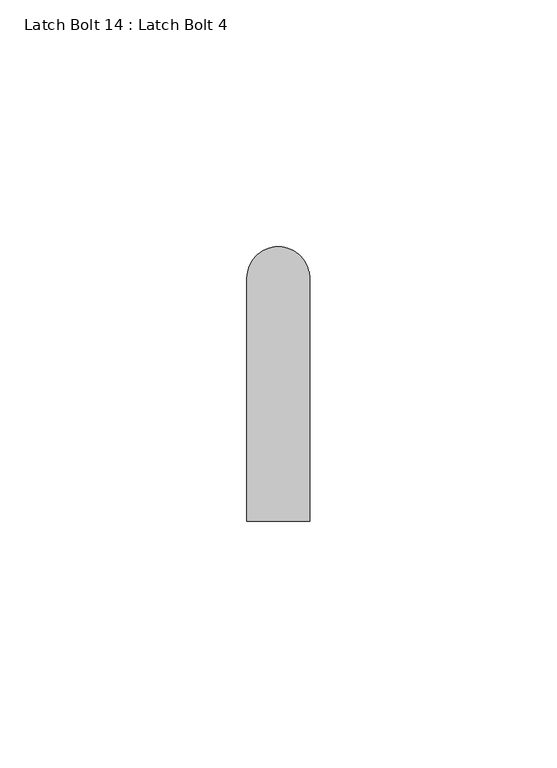
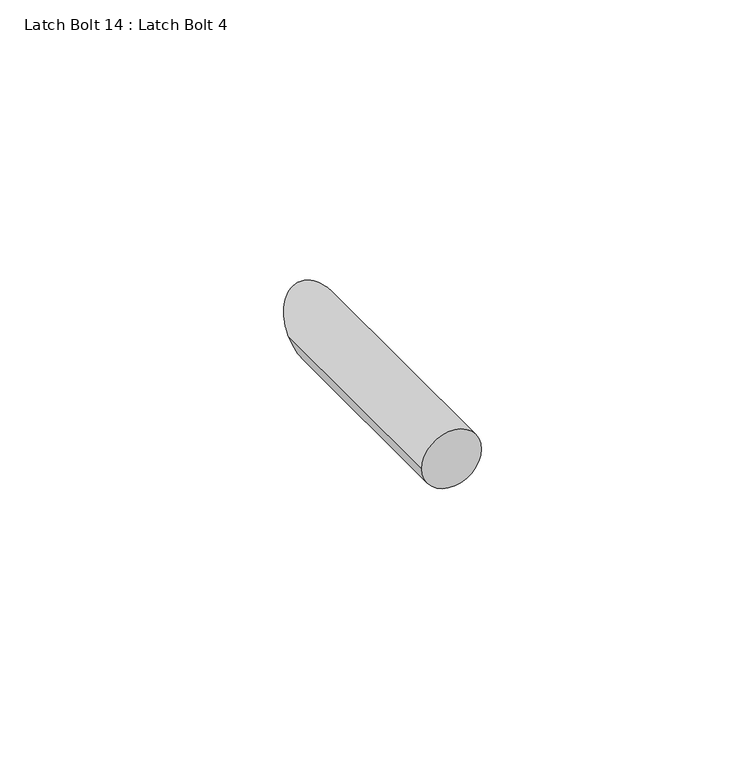
"""IFC4 building model written with IfcOpenShell, lengths in millimetres: proxy geometry, Latch Bolt 14 : Latch Bolt 4."""

from ifc_helpers import new_model, si_unit, frame, origin, place, context, project, spatial, circle_curve, ellipse_curve, source, transform, mapped, element, save
from ifc_brep_helpers import plane_surface, cylinder_surface, advanced_brep


def latch_bolt_14_latch_bolt_4_7b3a1efd(model_context):
    return source(origin(), model_context, "Body", "AdvancedBrep", [
        advanced_brep(
        [(587315.8935739, -535212.6610985, 292.1), (587303.1935739, -535212.6610985, 292.1), (587315.8935739, -535163.4485985, 292.1), (587303.1935739, -535163.4485985, 292.1)],
        [
            (0, 1, circle_curve(frame((587309.5435739, -535212.6610985, 292.1), z_axis=(0.0, -1.0, 0.0), x_axis=(1.0, 0.0, 0.0)), 6.35)),
            (1, 0, circle_curve(frame((587309.5435739, -535212.6610985, 292.1), z_axis=(0.0, -1.0, 0.0), x_axis=(1.0, 0.0, 0.0)), 6.35)),
            (0, 2),
            (2, 3, ellipse_curve(frame((587309.5435739, -535163.4485985, 292.1), z_axis=(0.0, -0.7071067811865497, 0.7071067811865455), x_axis=(0.0, -0.7071067811865454, -0.7071067811865497)), 8.9802561, 6.35)),
            (3, 1),
            (3, 2, ellipse_curve(frame((587309.5435739, -535163.4485985, 292.1), z_axis=(0.0, -0.7071067811865497, 0.7071067811865455), x_axis=(0.0, -0.7071067811865454, -0.7071067811865497)), 8.9802561, 6.35)),
        ],
        [
            plane_surface(frame((587315.8935739, -535212.6610985, 292.1), z_axis=(0.0, -1.0, 0.0), x_axis=(0.0, 0.0, 1.0))),
            cylinder_surface(frame((587309.5435739, -535155.5110985, 292.1), z_axis=(0.0, -1.0, 0.0), x_axis=(1.0, 0.0, 0.0)), 6.35),
            plane_surface(frame((587338.1185739, -535171.3860985, 284.1625), z_axis=(0.0, 0.7071067811865497, -0.7071067811865455), x_axis=(-1.0, 0.0, 0.0))),
        ],
        [
            (0, [[1, 2]]),
            (1, [[-1, 3, 4, 5]]),
            (1, [[-2, -5, 6, -3]]),
            (2, [[-4, -6]]),
        ],
    ),
    ])


if __name__ == "__main__":
    model = new_model("IFC4")
    model_context = context("Model", 3, world=origin())
    ifc_project = project(units=[si_unit("LENGTHUNIT", "METRE", prefix="MILLI")], contexts=[model_context])
    site = spatial("IfcSite", under=ifc_project)
    building = spatial("IfcBuilding", under=site)
    placement = place(None, origin())
    latch_bolt_14_latch_bolt_4_shape = latch_bolt_14_latch_bolt_4_7b3a1efd(model_context)
    element("IfcBuildingElementProxy", 1, Name="Latch Bolt 14 : Latch Bolt 4", ObjectType="Latch Bolt 14 : Latch Bolt 4", at=placement, inside=building, context=model_context, shape_type="MappedRepresentation", body=[
        mapped(latch_bolt_14_latch_bolt_4_shape, transform((0.0, 0.0, 0.0), x_axis=(1.0, 0.0, 0.0), y_axis=(0.0, 1.0, 0.0), z_axis=(0.0, 0.0, 1.0))),
    ])
    save(model, "model.ifc")

# Revit data of these elements
# Element 1 (IfcBuildingElementProxy, "Latch Bolt 14 : Latch Bolt 4")
#   Materials on its faces: "GALV. SLIDE BOLT"
# Materials
#   "GALV. SLIDE BOLT": class "Metal", colour RGB 189 187 185, transparency 0, Description = "Carbon steel", Cost = 0
